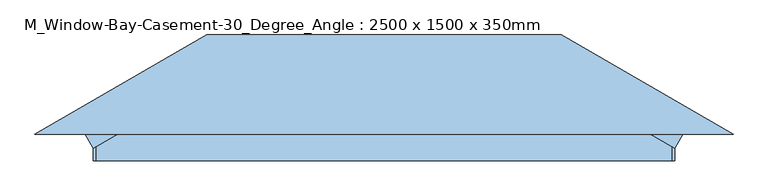
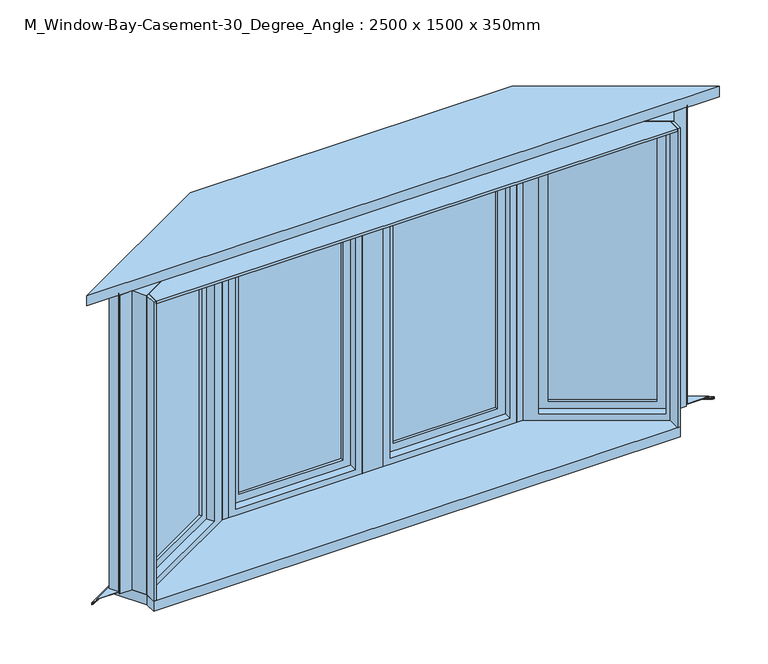
"""IFC4 building model written with IfcOpenShell, lengths in millimetres: window geometry, M_Window-Bay-Casement-30_Degree_Angle : 2500 x 1500 x 350mm."""

from ifc_helpers import new_model, si_unit, frame, origin, place, context, project, spatial, polyline, outline, extrude, faceted_brep, source, transform, mapped, element, save


def m_window_bay_casement_30_degree_angle_2500_x_1500_x_350mm_0d4230c8(model_context):
    return source(origin(), model_context, "Body", "SolidModel", [
        extrude(outline(polyline([(1224.4331255, 92.425), (1221.2581255, 86.9257387), (835.0107955, 309.9257387), (838.1857955, 315.425), (1224.4331255, 92.425)])), frame((0.0, 0.0, 720.65), z_axis=(0.0, 0.0, 1.0), x_axis=(1.0, 0.0, 0.0)), (0.0, 0.0, 1.0), 1360.3),
        extrude(outline(polyline([(1218.0831255, 81.4264774), (1214.9081255, 75.9272161), (828.6607955, 298.9272161), (831.8357955, 304.4264774), (1218.0831255, 81.4264774)])), frame((0.0, 0.0, 720.65), z_axis=(0.0, 0.0, 1.0), x_axis=(1.0, 0.0, 0.0)), (0.0, 0.0, 1.0), 1360.3),
        extrude(outline(polyline([(1417.45, 57.1500001), (1417.45, -503.15), (-57.15, -503.15), (-57.15, 57.1500001), (1417.45, 57.1500001)]), holes=[polyline([(1360.3, -445.9999999), (1360.3, 0.0), (0.0, 0.0), (0.0, -445.9999999), (1360.3, -445.9999999)])]), frame((1208.5581255, 64.9286934, 720.65), z_axis=(0.49999999999999967, 0.8660254037844388, 0.0), x_axis=(0.0, 0.0, 1.0)), (0.0, 0.0, 1.0), 44.45),
        faceted_brep([(714.9835794, 305.9, 2150.8), (1250.0, -2.9918745, 2150.8), (1284.925, 57.5, 2150.8), (1344.7940905, 57.5, 2150.8), (1344.7940905, 59.5963066, 2150.8), (742.2072174, 407.5, 2150.8), (1258.0514774, 36.3536934, 2138.1), (772.8174436, 316.5036934, 2138.1), (804.5674436, 371.4963066, 2138.1), (1289.8014774, 91.3463066, 2138.1), (1222.5036934, 12.8831255, 2119.05), (770.2652276, 273.9831255, 2119.05), (789.3152276, 306.9786934, 2119.05), (1241.5536934, 45.8786934, 2119.05), (772.8174436, 316.5036934, 663.5), (804.5674436, 371.4963066, 663.5), (770.2652276, 273.9831255, 682.55), (789.3152276, 306.9786934, 682.55), (742.2072174, 407.5, 650.8), (1344.7940905, 59.5963066, 650.8), (1344.7940905, 57.5, 650.8), (1284.925, 57.5, 650.8), (1250.0, -2.9918745, 650.8), (714.9835794, 305.9, 650.8), (1258.0514774, 36.3536934, 663.5), (1289.8014774, 91.3463066, 663.5), (1222.5036934, 12.8831255, 682.55), (1241.5536934, 45.8786934, 682.55)], [[[0, 1, 2, 3, 4, 5]], [[6, 7, 8, 9]], [[10, 11, 12, 13]], [[7, 14, 15, 8]], [[11, 16, 17, 12]], [[18, 19, 20, 21, 22, 23]], [[14, 24, 25, 15]], [[16, 26, 27, 17]], [[22, 21, 2, 1]], [[4, 19, 18, 5], [8, 15, 25, 9]], [[9, 25, 24, 6]], [[6, 24, 14, 7], [12, 17, 27, 13]], [[13, 27, 26, 10]], [[1, 0, 23, 22], [10, 26, 16, 11]], [[5, 18, 23, 0]], [[2, 21, 20, 3]], [[3, 20, 19, 4]]]),
        extrude(outline(polyline([(-1224.4331255, 92.425), (-838.1857955, 315.425), (-835.0107955, 309.9257387), (-1221.2581255, 86.9257387), (-1224.4331255, 92.425)])), frame((0.0, 0.0, 720.65), z_axis=(0.0, 0.0, 1.0), x_axis=(1.0, 0.0, 0.0)), (0.0, 0.0, 1.0), 1360.3),
        extrude(outline(polyline([(-1218.0831255, 81.4264774), (-831.8357955, 304.4264774), (-828.6607955, 298.9272161), (-1214.9081255, 75.9272161), (-1218.0831255, 81.4264774)])), frame((0.0, 0.0, 720.65), z_axis=(0.0, 0.0, 1.0), x_axis=(1.0, 0.0, 0.0)), (0.0, 0.0, 1.0), 1360.3),
        extrude(outline(polyline([(1417.45, -57.1500001), (-57.15, -57.1500001), (-57.15, 503.15), (1417.45, 503.15), (1417.45, -57.1500001)]), holes=[polyline([(1360.3, 445.9999999), (0.0, 445.9999999), (0.0, 0.0), (1360.3, 0.0), (1360.3, 445.9999999)])]), frame((-1208.5581255, 64.9286934, 720.65), z_axis=(-0.49999999999999967, 0.8660254037844388, 0.0), x_axis=(0.0, 0.0, 1.0)), (0.0, 0.0, 1.0), 44.45),
        faceted_brep([(-714.9835794, 305.9, 2150.8), (-742.2072174, 407.5, 2150.8), (-1344.7940905, 59.5963066, 2150.8), (-1344.7940905, 57.5, 2150.8), (-1284.925, 57.5, 2150.8), (-1250.0, -2.9918745, 2150.8), (-1258.0514774, 36.3536934, 2138.1), (-1289.8014774, 91.3463066, 2138.1), (-804.5674436, 371.4963066, 2138.1), (-772.8174436, 316.5036934, 2138.1), (-1222.5036934, 12.8831255, 2119.05), (-1241.5536934, 45.8786934, 2119.05), (-789.3152276, 306.9786934, 2119.05), (-770.2652276, 273.9831255, 2119.05), (-804.5674436, 371.4963066, 663.5), (-772.8174436, 316.5036934, 663.5), (-789.3152276, 306.9786934, 682.55), (-770.2652276, 273.9831255, 682.55), (-742.2072174, 407.5, 650.8), (-714.9835794, 305.9, 650.8), (-1250.0, -2.9918745, 650.8), (-1284.925, 57.5, 650.8), (-1344.7940905, 57.5, 650.8), (-1344.7940905, 59.5963066, 650.8), (-1289.8014774, 91.3463066, 663.5), (-1258.0514774, 36.3536934, 663.5), (-1241.5536934, 45.8786934, 682.55), (-1222.5036934, 12.8831255, 682.55)], [[[0, 1, 2, 3, 4, 5]], [[6, 7, 8, 9]], [[10, 11, 12, 13]], [[9, 8, 14, 15]], [[13, 12, 16, 17]], [[18, 19, 20, 21, 22, 23]], [[15, 14, 24, 25]], [[17, 16, 26, 27]], [[20, 5, 4, 21]], [[2, 1, 18, 23], [8, 7, 24, 14]], [[7, 6, 25, 24]], [[6, 9, 15, 25], [12, 11, 26, 16]], [[11, 10, 27, 26]], [[5, 20, 19, 0], [10, 13, 17, 27]], [[1, 0, 19, 18]], [[4, 3, 22, 21]], [[3, 2, 23, 22]]]),
        faceted_brep([(-755.844462, 458.3, 660.4), (-755.844462, 458.3, 653.0697935), (755.844462, 458.3, 653.0697935), (755.844462, 458.3, 660.4), (-742.232643, 407.5, 663.1486341), (-742.232643, 407.5, 660.4), (742.232643, 407.5, 660.4), (742.232643, 407.5, 663.1486341), (-756.218787, 459.697, 654.4483503), (-756.218787, 459.697, 663.1486341), (756.218787, 459.697, 663.1486341), (756.218787, 459.697, 654.4483503), (759.6217417, 472.397, 652.2089977), (-759.6217417, 472.397, 652.2089977), (759.6217417, 472.397, 643.2668038), (-759.6217417, 472.397, 643.2668038), (-758.5600199, 468.4346, 644.7270038), (-758.5600199, 468.4346, 643.2668038), (758.5600199, 468.4346, 643.2668038), (758.5600199, 468.4346, 644.7270038), (-759.1929694, 470.7968, 650.8662705), (-759.1929694, 470.7968, 644.7270038), (759.1929694, 470.7968, 644.7270038), (759.1929694, 470.7968, 650.8662705), (-1450.0504256, 57.5, 660.4), (-1450.0504256, 57.5, 653.0697935), (1450.0504256, 57.5, 660.4), (1348.4504256, 57.5, 660.4), (-1348.4504256, 57.5, 660.4), (-1348.4504256, 57.5, 663.1486341), (1348.4504256, 57.5, 663.1486341), (1452.8444256, 57.5, 663.1486341), (-1452.8444256, 57.5, 663.1486341), (-1452.8444256, 57.5, 654.4483503), (-1478.2444256, 57.5, 652.2089977), (-1478.2444256, 57.5, 643.2668038), (1478.2444256, 57.5, 643.2668038), (1470.3196257, 57.5, 643.2668038), (-1470.3196257, 57.5, 643.2668038), (-1470.3196257, 57.5, 644.7270038), (1470.3196257, 57.5, 644.7270038), (1475.0440256, 57.5, 644.7270038), (-1475.0440256, 57.5, 644.7270038), (-1475.0440256, 57.5, 650.8662705), (1450.0504256, 57.5, 653.0697935), (1452.8444256, 57.5, 654.4483503), (1478.2444256, 57.5, 652.2089977), (1475.0440256, 57.5, 650.8662705)], [[[0, 1, 2, 3]], [[4, 5, 6, 7]], [[8, 9, 10, 11]], [[8, 11, 12, 13]], [[13, 12, 14, 15]], [[16, 17, 18, 19]], [[20, 21, 22, 23]], [[2, 1, 20, 23]], [[1, 0, 24, 25]], [[0, 3, 26, 27, 6, 5, 28, 24]], [[5, 4, 29, 28]], [[4, 7, 30, 31, 10, 9, 32, 29]], [[9, 8, 33, 32]], [[8, 13, 34, 33]], [[13, 15, 35, 34]], [[15, 14, 36, 37, 18, 17, 38, 35]], [[17, 16, 39, 38]], [[16, 19, 40, 41, 22, 21, 42, 39]], [[21, 20, 43, 42]], [[20, 1, 25, 43]], [[3, 2, 44, 26]], [[7, 6, 27, 30]], [[11, 10, 31, 45]], [[12, 11, 45, 46]], [[14, 12, 46, 36]], [[19, 18, 37, 40]], [[23, 22, 41, 47]], [[2, 23, 47, 44]], [[25, 24, 28, 29, 32, 33, 34, 35, 38, 39, 42, 43]], [[27, 26, 44, 47, 41, 40, 37, 36, 46, 45, 31, 30]]]),
        extrude(outline(polyline([(-1320.9541191, 73.375), (-1348.4504256, 57.5), (-1370.6754256, 95.9948292), (-1343.1791191, 111.8698292), (-1320.9541191, 73.375)])), frame((0.0, 0.0, 663.1486341), z_axis=(0.0, 0.0, 1.0), x_axis=(1.0, 0.0, 0.0)), (0.0, 0.0, 1.0), 1497.2513659),
        extrude(outline(polyline([(1320.9541191, 73.375), (1343.1791191, 111.8698292), (1370.6754256, 95.9948292), (1348.4504256, 57.5), (1320.9541191, 73.375)])), frame((0.0, 0.0, 663.1486341), z_axis=(0.0, 0.0, 1.0), x_axis=(1.0, 0.0, 0.0)), (0.0, 0.0, 1.0), 1497.2513659),
        extrude(outline(polyline([(-714.9835794, 305.9), (714.9835794, 305.9), (1237.3, 4.340474), (1237.3, -57.5), (-1237.3, -57.5), (-1237.3, 4.340474), (-714.9835794, 305.9)])), frame((0.0, 0.0, 2138.1), z_axis=(0.0, 0.0, 1.0), x_axis=(1.0, 0.0, 0.0)), (0.0, 0.0, 1.0), 12.7),
        extrude(outline(polyline([(-1250.0, -57.5), (-1250.0, -2.9918745), (-1237.3, 4.340474), (-1237.3, -57.5), (-1250.0, -57.5)])), frame((0.0, 0.0, 650.8), z_axis=(0.0, 0.0, 1.0), x_axis=(1.0, 0.0, 0.0)), (0.0, 0.0, 1.0), 1500.0),
        extrude(outline(polyline([(1250.0, -57.5), (1237.3, -57.5), (1237.3, 4.340474), (1250.0, -2.9918744), (1250.0, -57.5)])), frame((0.0, 0.0, 650.8), z_axis=(0.0, 0.0, 1.0), x_axis=(1.0, 0.0, 0.0)), (0.0, 0.0, 1.0), 1500.0),
        extrude(outline(polyline([(2138.1, -670.1998305), (663.5, -670.1998305), (663.5, -63.5), (2138.1, -63.5), (2138.1, -670.1998305)]), holes=[polyline([(2080.95, -120.65), (720.65, -120.65), (720.65, -613.0498305), (2080.95, -613.0498305), (2080.95, -120.65)])]), frame((0.0, 344.0, 0.0), z_axis=(0.0, 1.0, 0.0), x_axis=(0.0, 0.0, 1.0)), (0.0, 0.0, 1.0), 44.45),
        extrude(outline(polyline([(2138.1, 63.5), (663.5, 63.5), (663.5, 670.1998305), (2138.1, 670.1998305), (2138.1, 63.5)]), holes=[polyline([(2080.95, 613.0498305), (720.65, 613.0498305), (720.65, 120.65), (2080.95, 120.65), (2080.95, 613.0498305)])]), frame((0.0, 344.0, 0.0), z_axis=(0.0, 1.0, 0.0), x_axis=(0.0, 0.0, 1.0)), (0.0, 0.0, 1.0), 44.45),
        extrude(outline(polyline([(1250.0, -57.5), (-1250.0, -57.5), (-1250.0, -2.9918745), (-1326.2, 128.9903971), (-755.8190363, 458.3), (755.8190363, 458.3), (1326.2, 128.9903971), (1250.0, -2.9918744), (1250.0, -57.5)])), frame((0.0, 0.0, 600.0), z_axis=(0.0, 0.0, 1.0), x_axis=(1.0, 0.0, 0.0)), (0.0, 0.0, 1.0), 50.8),
        faceted_brep([(670.1998305, 344.0, 663.5), (670.1998305, 407.5, 663.5), (63.5, 407.5, 663.5), (63.5, 344.0, 663.5), (651.1498305, 305.9, 682.55), (651.1498305, 344.0, 682.55), (82.55, 344.0, 682.55), (82.55, 305.9, 682.55), (682.8998305, 407.5, 650.8), (682.8998305, 305.9, 650.8), (50.8, 305.9, 650.8), (50.8, 407.5, 650.8), (63.5, 407.5, 2138.1), (63.5, 344.0, 2138.1), (82.55, 344.0, 2119.05), (82.55, 305.9, 2119.05), (50.8, 305.9, 2150.8), (50.8, 407.5, 2150.8), (670.1998305, 407.5, 2138.1), (670.1998305, 344.0, 2138.1), (651.1498305, 344.0, 2119.05), (651.1498305, 305.9, 2119.05), (682.8998305, 305.9, 2150.8), (682.8998305, 407.5, 2150.8)], [[[0, 1, 2, 3]], [[4, 5, 6, 7]], [[8, 9, 10, 11]], [[3, 2, 12, 13]], [[7, 6, 14, 15]], [[11, 10, 16, 17]], [[13, 12, 18, 19]], [[15, 14, 20, 21]], [[17, 16, 22, 23]], [[11, 17, 23, 8], [1, 18, 12, 2]], [[19, 18, 1, 0]], [[3, 13, 19, 0], [5, 20, 14, 6]], [[21, 20, 5, 4]], [[9, 22, 16, 10], [7, 15, 21, 4]], [[23, 22, 9, 8]]]),
        extrude(outline(polyline([(613.0498305, 375.75), (613.0498305, 369.4), (120.65, 369.4), (120.65, 375.75), (613.0498305, 375.75)])), frame((0.0, 0.0, 720.65), z_axis=(0.0, 0.0, 1.0), x_axis=(1.0, 0.0, 0.0)), (0.0, 0.0, 1.0), 1360.3),
        extrude(outline(polyline([(613.0498305, 363.05), (613.0498305, 356.7), (120.65, 356.7), (120.65, 363.05), (613.0498305, 363.05)])), frame((0.0, 0.0, 720.65), z_axis=(0.0, 0.0, 1.0), x_axis=(1.0, 0.0, 0.0)), (0.0, 0.0, 1.0), 1360.3),
        extrude(outline(polyline([(-120.65, 375.75), (-120.65, 369.4), (-613.0498305, 369.4), (-613.0498305, 375.75), (-120.65, 375.75)])), frame((0.0, 0.0, 720.65), z_axis=(0.0, 0.0, 1.0), x_axis=(1.0, 0.0, 0.0)), (0.0, 0.0, 1.0), 1360.3),
        extrude(outline(polyline([(-120.65, 363.05), (-120.65, 356.7), (-613.0498305, 356.7), (-613.0498305, 363.05), (-120.65, 363.05)])), frame((0.0, 0.0, 720.65), z_axis=(0.0, 0.0, 1.0), x_axis=(1.0, 0.0, 0.0)), (0.0, 0.0, 1.0), 1360.3),
        faceted_brep([(-63.5, 344.0, 663.5), (-63.5, 407.5, 663.5), (-670.1998305, 407.5, 663.5), (-670.1998305, 344.0, 663.5), (-82.55, 305.9, 682.55), (-82.55, 344.0, 682.55), (-651.1498305, 344.0, 682.55), (-651.1498305, 305.9, 682.55), (-50.8, 407.5, 650.8), (-50.8, 305.9, 650.8), (-682.8998305, 305.9, 650.8), (-682.8998305, 407.5, 650.8), (-670.1998305, 407.5, 2138.1), (-670.1998305, 344.0, 2138.1), (-651.1498305, 344.0, 2119.05), (-651.1498305, 305.9, 2119.05), (-682.8998305, 305.9, 2150.8), (-682.8998305, 407.5, 2150.8), (-63.5, 407.5, 2138.1), (-63.5, 344.0, 2138.1), (-82.55, 344.0, 2119.05), (-82.55, 305.9, 2119.05), (-50.8, 305.9, 2150.8), (-50.8, 407.5, 2150.8)], [[[0, 1, 2, 3]], [[4, 5, 6, 7]], [[8, 9, 10, 11]], [[3, 2, 12, 13]], [[7, 6, 14, 15]], [[11, 10, 16, 17]], [[13, 12, 18, 19]], [[15, 14, 20, 21]], [[17, 16, 22, 23]], [[11, 17, 23, 8], [1, 18, 12, 2]], [[19, 18, 1, 0]], [[3, 13, 19, 0], [5, 20, 14, 6]], [[21, 20, 5, 4]], [[9, 22, 16, 10], [7, 15, 21, 4]], [[23, 22, 9, 8]]]),
        extrude(outline(polyline([(50.8, 407.5), (50.8, 305.9), (-50.8, 305.9), (-50.8, 407.5), (50.8, 407.5)])), frame((0.0, 0.0, 650.8), z_axis=(0.0, 0.0, 1.0), x_axis=(1.0, 0.0, 0.0)), (0.0, 0.0, 1.0), 1500.0),
        extrude(outline(polyline([(-682.8998305, 407.5), (-682.8998305, 305.9), (-714.9835794, 305.9), (-742.2072173, 407.5), (-682.8998305, 407.5)])), frame((0.0, 0.0, 650.8), z_axis=(0.0, 0.0, 1.0), x_axis=(1.0, 0.0, 0.0)), (0.0, 0.0, 1.0), 1500.0),
        extrude(outline(polyline([(742.2072173, 407.5), (714.9835794, 305.9), (682.8998305, 305.9), (682.8998305, 407.5), (742.2072173, 407.5)])), frame((0.0, 0.0, 650.8), z_axis=(0.0, 0.0, 1.0), x_axis=(1.0, 0.0, 0.0)), (0.0, 0.0, 1.0), 1500.0),
        extrude(outline(polyline([(762.6249458, 483.7), (1500.825, 57.5), (-1500.825, 57.5), (-762.6249458, 483.7), (762.6249458, 483.7)])), frame((0.0, 0.0, 2150.8), z_axis=(0.0, 0.0, 1.0), x_axis=(1.0, 0.0, 0.0)), (0.0, 0.0, 1.0), 50.8),
    ])


if __name__ == "__main__":
    model = new_model("IFC4")
    model_context = context("Model", 3, world=origin())
    ifc_project = project(units=[si_unit("LENGTHUNIT", "METRE", prefix="MILLI")], contexts=[model_context])
    site = spatial("IfcSite", under=ifc_project)
    building = spatial("IfcBuilding", under=site)
    placement = place(None, origin())
    m_window_bay_casement_30_degree_angle_2500_x_1500_x_350mm_shape = m_window_bay_casement_30_degree_angle_2500_x_1500_x_350mm_0d4230c8(model_context)
    element("IfcWindow", 1, ObjectType="M_Window-Bay-Casement-30_Degree_Angle : 2500 x 1500 x 350mm", at=placement, inside=building, context=model_context, shape_type="MappedRepresentation", body=[
        mapped(m_window_bay_casement_30_degree_angle_2500_x_1500_x_350mm_shape, transform((0.0, 0.0, 0.0), x_axis=(1.0, 0.0, 0.0), y_axis=(0.0, 1.0, 0.0), z_axis=(0.0, 0.0, 1.0))),
    ])
    save(model, "model.ifc")

# Revit data of these elements
# Type "M_Window-Bay-Casement-30_Degree_Angle : 2500 x 1500 x 350mm"
#   Type Mark = "50"
#   Fire Rating = "0.5h"
#   Assembly Code = "B2020100"
#   Analytic Construction = "Double glazing - domestic"
#   Width of Middle Sash = 1365.8 mm
#   Width = 2500 mm
#   Visual Light Transmittance = 0.81
#   Thermal Resistance (R) = 0.319569 (m²·K)/W
#   Solar Heat Gain Coefficient = 0.76
#   Rough Width = 2515 mm
#   Rough Height = 1515 mm
#   Length 2 = 1484.465 mm
#   Length 1 = 516.3 mm
#   Wall Thickness [instance default] = 150 mm
#   Trim Width = 2618.666 mm
#   Trim Height = 1500 mm
#   Height 1 = 1550.8 mm
#   Height = 1500 mm
#   Heat Transfer Coefficient (U) = 3.12929 W/(m²·K)
#   Depth = 350 mm
#   Default Sill Height = 600 mm
#   Angle = 30.00°
#   Muntin Visibility = yes
#   Interior Trim Visibility [instance default] = yes
#   Exterior Trim Visibility [instance default] = yes
#   Muntin Pattern = M_Muntin Pattern_2x2 : M_Muntin Pattern_2x2
#   Interior Trim Material = Wood - Stained
#   Exterior Trim Material = Clad - White
#   Exterior Trim = element 343235
#   Interior Trim = M_Trim-Window-Interior-Flat : Picture Frame
#   Interior Frame Material = Wood - Stained
#   Glass Panel Material = Glass
#   Exterior Frame Material = Clad - White
#   Wall Closure = (empty or 0)
# Element 1 (IfcWindow, "M_Window-Bay-Casement-30_Degree_Angle : 2500 x 1500 x 350mm")
#   Wall Thickness = 115 mm
#   Materials on its faces: "Clad - White", "Wood - Stained", "Glass"
# Materials
#   "Wood - Stained": class "Wood", colour RGB 227 170 128, transparency 0, Cost = 0
#   "Clad - White": class "Wood", colour RGB 242 242 238, transparency 0, Cost = 0
#   "Glass": class "Glass", colour RGB 0 128 192, transparency 0.9, Description = "Soda Lime Glass", Cost = 0
